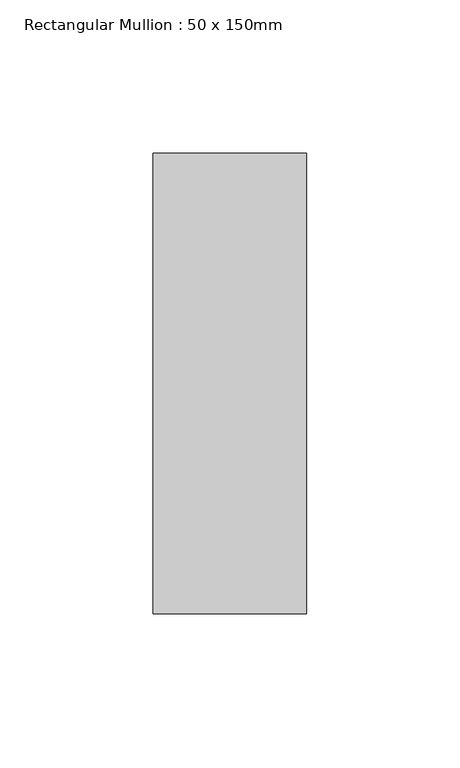
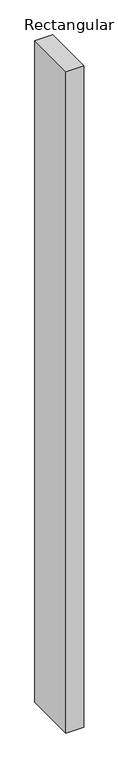
"""IFC4 building model written with IfcOpenShell, lengths in millimetres: member geometry, Rectangular Mullion : 50 x 150mm."""

from ifc_helpers import new_model, si_unit, frame, origin, place, context, project, spatial, polyline, outline, extrude, source, transform, mapped, element, save


def rectangular_mullion_50_x_150mm_0967fd3c(model_context):
    return source(origin(), model_context, "Body", "SweptSolid", [
        extrude(outline(polyline([(0.0, 75.0), (0.0, -75.0), (-50.0, -75.0), (-50.0, 75.0), (0.0, 75.0)])), frame((0.0, 0.0, -1950.0000003), z_axis=(0.0, 0.0, 1.0), x_axis=(1.0, 0.0, 0.0)), (0.0, 0.0, 1.0), 1950.0000003),
    ])


if __name__ == "__main__":
    model = new_model("IFC4")
    model_context = context("Model", 3, world=origin())
    ifc_project = project(units=[si_unit("LENGTHUNIT", "METRE", prefix="MILLI")], contexts=[model_context])
    site = spatial("IfcSite", under=ifc_project)
    building = spatial("IfcBuilding", under=site)
    placement = place(None, origin())
    rectangular_mullion_50_x_150mm_shape = rectangular_mullion_50_x_150mm_0967fd3c(model_context)
    element("IfcMember", 1, ObjectType="Rectangular Mullion : 50 x 150mm", at=placement, inside=building, context=model_context, shape_type="MappedRepresentation", body=[
        mapped(rectangular_mullion_50_x_150mm_shape, transform((0.0, 0.0, 0.0), x_axis=(1.0, 0.0, 0.0), y_axis=(0.0, 1.0, 0.0), z_axis=(0.0, 0.0, 1.0))),
    ])
    save(model, "model.ifc")

# Revit data of these elements
# Type "Rectangular Mullion : 50 x 150mm"
#   built-in parameter 1007304 = 0.492126 (stored number, unit not read)
#   built-in parameter 1007301 = 0.082021 (stored number, unit not read)
#   built-in parameter 1007300 = 0.082021 (stored number, unit not read)
# Element 1 (IfcMember, "Rectangular Mullion : 50 x 150mm")
#   Materials on its faces: "Metal - Aluminium"
# Materials
#   "Metal - Aluminium": class "Metal", colour RGB 247 247 247, transparency 0
